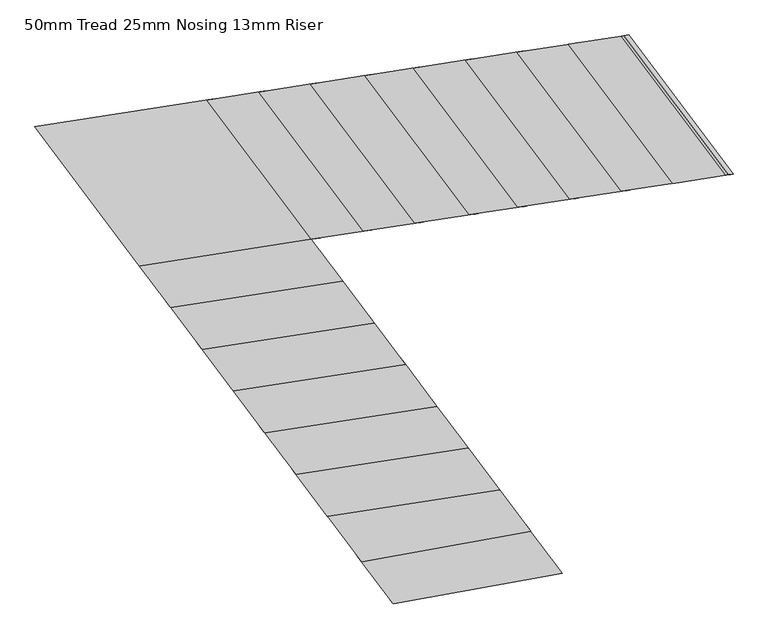
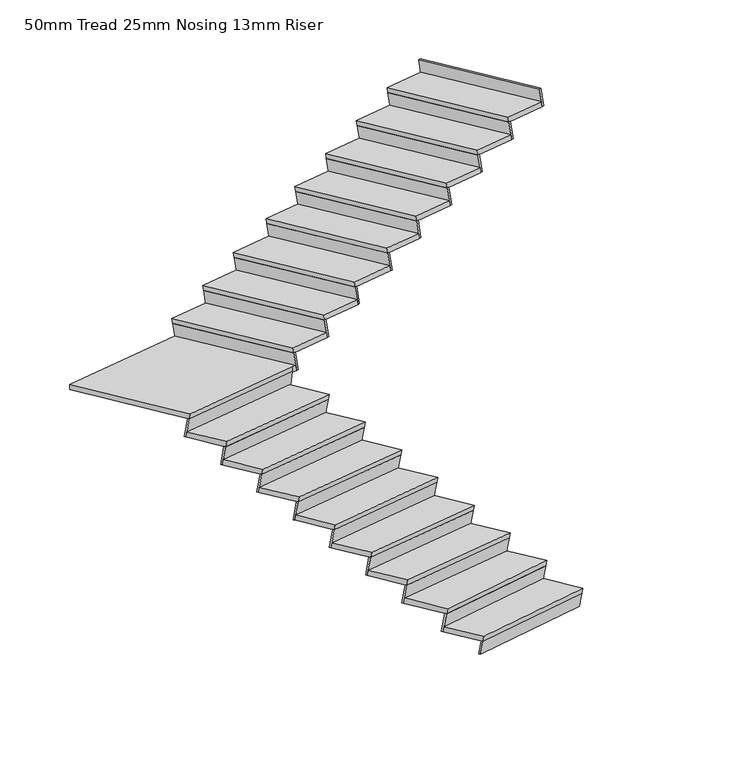
"""IFC4 building model written with IfcOpenShell, lengths in millimetres: stair flight geometry, 50mm Tread 25mm Nosing 13mm Riser."""

import ifcopenshell
import ifcopenshell.guid

model = None  # the IFC model being written
_history = None  # IfcOwnerHistory: only IFC2X3 demands one
_inside = {}  # id of a spatial element -> (the spatial element, [elements in it])
_under = {}  # id of a project, library or spatial element -> (it, [spatial elements below it])
_declared = {}  # id of a project -> (the project, [libraries it declares])
_typed = {}  # id of a type object -> (the type object, [elements of that type])
_made_of = {}  # id of a material, layer set ... -> (it, [elements and type objects made of it])


def new_model(schema):
    """Start an empty IFC model of exactly this schema.

    Asked for "IFC4X3", IfcOpenShell would pick the latest addendum, in which some entities
    have other attributes; the version numbers below select the first issue.
    IFC2X3 requires an IfcOwnerHistory on every rooted entity: one is made here for all.
    """
    global model, _history
    if schema == "IFC4X3":
        model = ifcopenshell.file(schema_version=(4, 3, 0, 0))
    else:
        model = ifcopenshell.file(schema=schema)
    _inside.clear()
    _under.clear()
    _declared.clear()
    _typed.clear()
    _made_of.clear()
    _history = None
    if model.schema == "IFC2X3":
        org = make("IfcOrganization", Name="unknown")
        user = make(
            "IfcPersonAndOrganization",
            ThePerson=make("IfcPerson", FamilyName="unknown"),
            TheOrganization=org,
        )
        app = make(
            "IfcApplication",
            ApplicationDeveloper=org,
            Version="unknown",
            ApplicationFullName="unknown",
            ApplicationIdentifier="unknown",
        )
        _history = make(
            "IfcOwnerHistory",
            OwningUser=user,
            OwningApplication=app,
            ChangeAction="ADDED",
            CreationDate=0,
        )
    return model


def make(cls, **values):
    """One entity of the class cls with the attributes given. An attribute that is None is left unset."""
    return model.create_entity(
        cls, **{name: value for name, value in values.items() if value is not None}
    )


def rooted(cls, **values):
    """An entity with a GlobalId (a new one), such as an element, a storey or a relation."""
    return make(cls, GlobalId=ifcopenshell.guid.new(), OwnerHistory=_history, **values)


def si_unit(unit_type, name, prefix=None):
    """IfcSIUnit, for example si_unit("LENGTHUNIT", "METRE", prefix="MILLI")."""
    return make("IfcSIUnit", UnitType=unit_type, Prefix=prefix, Name=name)


def assignment(units):
    """IfcUnitAssignment: the units of a project."""
    return None if units is None else make("IfcUnitAssignment", Units=units)


def point(xyz):
    """IfcCartesianPoint."""
    return None if xyz is None else make("IfcCartesianPoint", Coordinates=xyz)


def direction(xyz):
    """IfcDirection."""
    return None if xyz is None else make("IfcDirection", DirectionRatios=xyz)


def frame(location, z_axis=None, x_axis=None):
    """IfcAxis2Placement3D, a coordinate frame: its origin and axes. An axis left out is left unset."""
    return make(
        "IfcAxis2Placement3D",
        Location=point(location),
        Axis=direction(z_axis),
        RefDirection=direction(x_axis),
    )


def origin():
    """The frame at (0, 0, 0) with its axes left unset."""
    return frame((0.0, 0.0, 0.0))


def place(relative_to, where):
    """IfcLocalPlacement: puts the frame where relative to a parent placement (None: the world)."""
    return make(
        "IfcLocalPlacement", PlacementRelTo=relative_to, RelativePlacement=where
    )


def context(
    kind, dimensions, precision=None, world=None, true_north=None, identifier=None
):
    """IfcGeometricRepresentationContext, for example the 3D "Model" context."""
    return make(
        "IfcGeometricRepresentationContext",
        ContextIdentifier=identifier,
        ContextType=kind,
        CoordinateSpaceDimension=dimensions,
        Precision=precision,
        WorldCoordinateSystem=world,
        TrueNorth=true_north,
    )


def project(units=None, contexts=None):
    """IfcProject with its units and contexts."""
    return rooted(
        "IfcProject",
        Name="project",
        RepresentationContexts=contexts,
        UnitsInContext=assignment(units),
    )


def spatial(cls, under=None, at=None, **own):
    """A site, building, storey or space (cls), placed at a placement, below another one or the project."""
    s = rooted(cls, ObjectPlacement=at, **own)
    if under is not None:
        _under.setdefault(under.id(), (under, []))[1].append(s)
    return s


def faces_of(points, faces, orient=None, outer=None):
    """IfcFace entities. A face is a list of loops; a loop is a list of indices into points, from 0.

    orient and outer hold one flag for each loop. By default every Orientation is true, the
    first loop of a face is its IfcFaceOuterBound and the others are IfcFaceBound.
    """
    made = []
    for i, loops in enumerate(faces):
        bounds = []
        for j, loop in enumerate(loops):
            is_outer = j == 0 if outer is None else outer[i][j]
            bounds.append(
                make(
                    "IfcFaceOuterBound" if is_outer else "IfcFaceBound",
                    Bound=make("IfcPolyLoop", Polygon=[points[k] for k in loop]),
                    Orientation=True if orient is None else orient[i][j],
                )
            )
        made.append(make("IfcFace", Bounds=bounds))
    return made


def faceted_brep(points, faces, orient=None, outer=None, voids=None):
    """IfcFacetedBrep: a solid bounded by flat faces; with voids (closed shells), ...WithVoids."""
    shared = [point(p) for p in points]
    hull = make("IfcClosedShell", CfsFaces=faces_of(shared, faces, orient, outer))
    if voids is None:
        return make("IfcFacetedBrep", Outer=hull)
    return make(
        "IfcFacetedBrepWithVoids",
        Outer=hull,
        Voids=[
            make(cls, CfsFaces=faces_of(shared, fs, o, b)) for cls, fs, o, b in voids
        ],
    )


def shape(context_of_items, identifier, shape_type, items):
    """IfcShapeRepresentation: the items that make up one representation, for example the "Body"."""
    return make(
        "IfcShapeRepresentation",
        ContextOfItems=context_of_items,
        RepresentationIdentifier=identifier,
        RepresentationType=shape_type,
        Items=items,
    )


def source(mapping_origin, context_of_items, identifier, shape_type, items):
    """IfcRepresentationMap: a shape defined once, which mapped items show again and again."""
    return make(
        "IfcRepresentationMap",
        MappingOrigin=mapping_origin,
        MappedRepresentation=shape(context_of_items, identifier, shape_type, items),
    )


def transform(
    local_origin,
    x_axis=None,
    y_axis=None,
    z_axis=None,
    scale=None,
    scale2=None,
    scale3=None,
    uniform=True,
):
    """IfcCartesianTransformationOperator3D, or its non-uniform kind. x_axis, y_axis, z_axis: its Axis1, 2, 3."""
    if uniform:
        return make(
            "IfcCartesianTransformationOperator3D",
            Axis1=direction(x_axis),
            Axis2=direction(y_axis),
            LocalOrigin=point(local_origin),
            Scale=scale,
            Axis3=direction(z_axis),
        )
    return make(
        "IfcCartesianTransformationOperator3DnonUniform",
        Axis1=direction(x_axis),
        Axis2=direction(y_axis),
        LocalOrigin=point(local_origin),
        Scale=scale,
        Axis3=direction(z_axis),
        Scale2=scale2,
        Scale3=scale3,
    )


def mapped(mapping_source, mapping_target):
    """IfcMappedItem: shows the shape of a source again, moved by a transform."""
    return make(
        "IfcMappedItem", MappingSource=mapping_source, MappingTarget=mapping_target
    )


def made_of(thing, what):
    """Note that an element or type object is made of a material, layer set ...; save() writes the relation."""
    if what is not None:
        _made_of.setdefault(what.id(), (what, []))[1].append(thing)
    return thing


def element(
    cls,
    number,
    at=None,
    inside=None,
    cuts=None,
    type_object=None,
    material=None,
    context=None,
    identifier="Body",
    shape_type=None,
    held_by="IfcProductDefinitionShape",
    body=None,
    shapes=None,
    **own,
):
    """One element of the class cls, such as IfcWall. Its Tag is "e" and its number.

    at: its placement. inside: the storey or other place that contains it. cuts: it is an
    opening in that element (IfcRelVoidsElement). A single representation is given by context,
    identifier, shape_type and body (its items); several are given by shapes. held_by: the class
    of the entity that holds the representations. save() writes the other relations.
    """
    e = rooted(cls, Tag="e%d" % number, ObjectPlacement=at, **own)
    if body is not None:
        shapes = [shape(context, identifier, shape_type, body)]
    if shapes is not None:
        e.Representation = make(held_by, Representations=shapes)
    if inside is not None:
        _inside.setdefault(inside.id(), (inside, []))[1].append(e)
    if cuts is not None:
        rooted(
            "IfcRelVoidsElement", RelatingBuildingElement=cuts, RelatedOpeningElement=e
        )
    if type_object is not None:
        _typed.setdefault(type_object.id(), (type_object, []))[1].append(e)
    return made_of(e, material)


def aggregate(whole, parts):
    """IfcRelAggregates: a whole, such as a stair, and the parts it consists of."""
    return rooted("IfcRelAggregates", RelatingObject=whole, RelatedObjects=parts)


def save(model, path):
    """Write the relations noted so far, then the file.

    IfcRelAggregates (storeys below a building ...), IfcRelContainedInSpatialStructure (elements
    in a storey), IfcRelDefinesByType, IfcRelAssociatesMaterial and IfcRelDeclares: one each for
    every whole, place, type object, material and project.
    """
    for whole, parts in _under.values():
        aggregate(whole, parts)
    for where, things in _inside.values():
        rooted(
            "IfcRelContainedInSpatialStructure",
            RelatedElements=things,
            RelatingStructure=where,
        )
    for kind, things in _typed.values():
        rooted("IfcRelDefinesByType", RelatedObjects=things, RelatingType=kind)
    for what, things in _made_of.values():
        rooted("IfcRelAssociatesMaterial", RelatedObjects=things, RelatingMaterial=what)
    for by, libraries in _declared.values():
        rooted("IfcRelDeclares", RelatingContext=by, RelatedDefinitions=libraries)
    model.write(path)


def stair_flight_50mm_tread_25mm_nosing_13mm_riser_716ff132(model_context):
    return source(origin(), model_context, "Body", "Brep", [
        faceted_brep([(80293.6777293, 43226.6486407, 17175.0), (80288.8810609, 43233.0418362, 17125.0), (79317.3439262, 43057.8753097, 17125.0), (79322.1405946, 43051.4821142, 17175.0), (79518.9714946, 42789.1378561, 17175.0), (80490.5086293, 42964.3043826, 17175.0), (80485.7119608, 42970.6975781, 17125.0), (79514.1748261, 42795.5310516, 17125.0)], [[[0, 1, 2, 3]], [[3, 4, 5, 0]], [[2, 1, 6, 7]], [[4, 3, 2, 7]], [[0, 5, 6, 1]], [[5, 4, 7, 6]]]),
        faceted_brep([(80485.7119608, 42970.6975781, 17125.0), (80473.7202897, 42986.6805669, 17000.0), (80465.2408978, 42997.9822466, 17000.0), (80477.2325689, 42981.9992578, 17125.0), (79514.1748261, 42795.5310516, 17125.0), (79505.6954342, 42806.8327314, 17125.0), (79493.703763, 42822.8157201, 17000.0), (79502.183155, 42811.5140404, 17000.0)], [[[0, 1, 2, 3]], [[4, 5, 6, 7]], [[1, 0, 4, 7]], [[2, 1, 7, 6]], [[3, 2, 6, 5]], [[0, 3, 5, 4]]]),
        faceted_brep([(80305.6694004, 43210.6656519, 17300.0), (80288.8810609, 43233.0418362, 17125.0), (80280.4016689, 43244.3435159, 17125.0), (80297.1900085, 43221.9673316, 17300.0), (79334.1322657, 43035.4991254, 17300.0), (79325.6528738, 43046.8008052, 17300.0), (79308.8645342, 43069.1769895, 17125.0), (79317.3439262, 43057.8753097, 17125.0)], [[[0, 1, 2, 3]], [[4, 5, 6, 7]], [[1, 0, 4, 7]], [[2, 1, 7, 6]], [[3, 2, 6, 5]], [[0, 3, 5, 4]]]),
        faceted_brep([(79125.1762587, 43314.0042212, 17350.0), (79338.9289342, 43029.1059299, 17350.0), (80310.4660689, 43204.2724564, 17350.0), (80113.4175257, 43466.9067982, 17350.0), (79120.3174064, 43320.4802978, 17300.0), (80108.5586735, 43473.3828748, 17300.0), (80305.6694004, 43210.6656519, 17300.0), (79334.1322657, 43035.4991254, 17300.0)], [[[0, 1, 2, 3]], [[4, 5, 6, 7]], [[1, 0, 4, 7]], [[3, 2, 6, 5]], [[3, 5, 4, 0]], [[2, 1, 7, 6]]]),
        faceted_brep([(80125.5646563, 43450.7166068, 17475.0), (80108.5586735, 43473.3828748, 17300.0), (80099.9693551, 43484.8310689, 17300.0), (80116.9753379, 43462.1648009, 17475.0), (79137.3233892, 43297.8140298, 17475.0), (79128.7340708, 43309.2622239, 17475.0), (79111.7280881, 43331.9284919, 17300.0), (79120.3174064, 43320.4802978, 17300.0)], [[[0, 1, 2, 3]], [[4, 5, 6, 7]], [[1, 0, 4, 7]], [[2, 1, 7, 6]], [[3, 2, 6, 5]], [[0, 3, 5, 4]]]),
        faceted_brep([(78945.1336983, 43553.972295, 17525.0), (79142.1822414, 43291.3379532, 17525.0), (80130.4235085, 43444.2405302, 17525.0), (79933.3749653, 43706.874872, 17525.0), (78940.274846, 43560.4483716, 17475.0), (79928.5161131, 43713.3509486, 17475.0), (80125.5646563, 43450.7166068, 17475.0), (79137.3233892, 43297.8140298, 17475.0)], [[[0, 1, 2, 3]], [[4, 5, 6, 7]], [[1, 0, 4, 7]], [[3, 2, 6, 5]], [[3, 5, 4, 0]], [[2, 1, 7, 6]]]),
        faceted_brep([(79945.5220959, 43690.6846806, 17650.0), (79928.5161131, 43713.3509486, 17475.0), (79919.9267947, 43724.7991427, 17475.0), (79936.9327775, 43702.1328747, 17650.0), (78957.2808288, 43537.7821036, 17650.0), (78948.6915104, 43549.2302977, 17650.0), (78931.6855277, 43571.8965657, 17475.0), (78940.274846, 43560.4483716, 17475.0)], [[[0, 1, 2, 3]], [[4, 5, 6, 7]], [[1, 0, 4, 7]], [[2, 1, 7, 6]], [[3, 2, 6, 5]], [[0, 3, 5, 4]]]),
        faceted_brep([(78765.0911379, 43793.9403688, 17700.0), (78962.139681, 43531.306027, 17700.0), (79950.3809481, 43684.208604, 17700.0), (79753.3324049, 43946.8429458, 17700.0), (78760.2322857, 43800.4164454, 17650.0), (79748.4735527, 43953.3190224, 17650.0), (79945.5220959, 43690.6846806, 17650.0), (78957.2808288, 43537.7821036, 17650.0)], [[[0, 1, 2, 3]], [[4, 5, 6, 7]], [[1, 0, 4, 7]], [[3, 2, 6, 5]], [[3, 5, 4, 0]], [[2, 1, 7, 6]]]),
        faceted_brep([(79765.4795355, 43930.6527544, 17825.0), (79748.4735527, 43953.3190224, 17650.0), (79739.8842343, 43964.7672165, 17650.0), (79756.8902171, 43942.1009485, 17825.0), (78777.2382684, 43777.7501774, 17825.0), (78768.64895, 43789.1983715, 17825.0), (78751.6429673, 43811.8646395, 17650.0), (78760.2322857, 43800.4164454, 17650.0)], [[[0, 1, 2, 3]], [[4, 5, 6, 7]], [[1, 0, 4, 7]], [[2, 1, 7, 6]], [[3, 2, 6, 5]], [[0, 3, 5, 4]]]),
        faceted_brep([(78585.0485775, 44033.9084426, 17875.0), (78782.0971206, 43771.2741008, 17875.0), (79770.3383877, 43924.1766778, 17875.0), (79573.2898445, 44186.8110196, 17875.0), (78580.1897253, 44040.3845192, 17825.0), (79568.4309923, 44193.2870962, 17825.0), (79765.4795355, 43930.6527544, 17825.0), (78777.2382684, 43777.7501774, 17825.0)], [[[0, 1, 2, 3]], [[4, 5, 6, 7]], [[1, 0, 4, 7]], [[3, 2, 6, 5]], [[3, 5, 4, 0]], [[2, 1, 7, 6]]]),
        faceted_brep([(79585.4369751, 44170.6208282, 18000.0), (79568.4309923, 44193.2870962, 17825.0), (79559.841674, 44204.7352904, 17825.0), (79576.8476567, 44182.0690223, 18000.0), (78597.195708, 44017.7182512, 18000.0), (78588.6063896, 44029.1664453, 18000.0), (78571.6004069, 44051.8327134, 17825.0), (78580.1897253, 44040.3845192, 17825.0)], [[[0, 1, 2, 3]], [[4, 5, 6, 7]], [[1, 0, 4, 7]], [[2, 1, 7, 6]], [[3, 2, 6, 5]], [[0, 3, 5, 4]]]),
        faceted_brep([(78405.0060171, 44273.8765164, 18050.0), (78602.0545602, 44011.2421746, 18050.0), (79590.2958273, 44164.1447516, 18050.0), (79393.2472842, 44426.7790934, 18050.0), (78400.1471649, 44280.352593, 18000.0), (79388.3884319, 44433.25517, 18000.0), (79585.4369751, 44170.6208282, 18000.0), (78597.195708, 44017.7182512, 18000.0)], [[[0, 1, 2, 3]], [[4, 5, 6, 7]], [[1, 0, 4, 7]], [[3, 2, 6, 5]], [[3, 5, 4, 0]], [[2, 1, 7, 6]]]),
        faceted_brep([(79405.3944147, 44410.588902, 18175.0), (79388.3884319, 44433.25517, 18000.0), (79379.7991136, 44444.7033642, 18000.0), (79396.8050963, 44422.0370962, 18175.0), (78417.1531476, 44257.686325, 18175.0), (78408.5638292, 44269.1345192, 18175.0), (78391.5578465, 44291.8007872, 18000.0), (78400.1471649, 44280.352593, 18000.0)], [[[0, 1, 2, 3]], [[4, 5, 6, 7]], [[1, 0, 4, 7]], [[2, 1, 7, 6]], [[3, 2, 6, 5]], [[0, 3, 5, 4]]]),
        faceted_brep([(78224.9634567, 44513.8445902, 18225.0), (78422.0119998, 44251.2102484, 18225.0), (79410.2532669, 44404.1128254, 18225.0), (79213.2047238, 44666.7471672, 18225.0), (78220.1046045, 44520.3206668, 18175.0), (79208.3458715, 44673.2232438, 18175.0), (79405.3944147, 44410.588902, 18175.0), (78417.1531476, 44257.686325, 18175.0)], [[[0, 1, 2, 3]], [[4, 5, 6, 7]], [[1, 0, 4, 7]], [[3, 2, 6, 5]], [[3, 5, 4, 0]], [[2, 1, 7, 6]]]),
        faceted_brep([(79225.3518543, 44650.5569758, 18350.0), (79208.3458715, 44673.2232438, 18175.0), (79199.7565532, 44684.671438, 18175.0), (79216.7625359, 44662.00517, 18350.0), (78237.1105872, 44497.6543988, 18350.0), (78228.5212688, 44509.102593, 18350.0), (78211.5152861, 44531.768861, 18175.0), (78220.1046045, 44520.3206668, 18175.0)], [[[0, 1, 2, 3]], [[4, 5, 6, 7]], [[1, 0, 4, 7]], [[2, 1, 7, 6]], [[3, 2, 6, 5]], [[0, 3, 5, 4]]]),
        faceted_brep([(78044.9208963, 44753.812664, 18400.0), (78241.9694394, 44491.1783222, 18400.0), (79230.2107065, 44644.0808992, 18400.0), (79033.1621634, 44906.715241, 18400.0), (78040.0620441, 44760.2887406, 18350.0), (79028.3033111, 44913.1913176, 18350.0), (79225.3518543, 44650.5569758, 18350.0), (78237.1105872, 44497.6543988, 18350.0)], [[[0, 1, 2, 3]], [[4, 5, 6, 7]], [[1, 0, 4, 7]], [[3, 2, 6, 5]], [[3, 5, 4, 0]], [[2, 1, 7, 6]]]),
        faceted_brep([(79049.0759849, 44891.1078392, 18525.0), (79045.2534204, 44915.8138709, 18350.0), (79043.3227338, 44928.2923013, 18350.0), (79047.1452983, 44903.5862696, 18525.0), (78057.0680268, 44737.6224726, 18525.0), (78048.4787085, 44749.0706668, 18525.0), (78031.4727257, 44771.7369348, 18350.0), (78040.0620441, 44760.2887406, 18350.0)], [[[0, 1, 2, 3]], [[4, 5, 6, 7]], [[1, 0, 4, 7]], [[2, 1, 7, 6]], [[3, 2, 6, 5]], [[0, 3, 5, 4]]]),
        faceted_brep([(78478.0296801, 45688.2752923, 18575.0), (77461.7850111, 45531.0399754, 18575.0), (78061.926879, 44731.146396, 18575.0), (79050.1681461, 44884.048973, 18575.0), (79078.1715481, 44888.3817129, 18575.0), (78486.0306521, 45689.5132179, 18525.0), (79086.17252, 44889.6196386, 18525.0), (79050.1681461, 44884.048973, 18525.0), (79049.0759849, 44891.1078392, 18525.0), (78057.0680268, 44737.6224726, 18525.0), (77461.7850111, 45531.0399754, 18525.0)], [[[0, 1, 2, 3, 4]], [[5, 6, 7, 8, 9, 10]], [[1, 0, 5, 10]], [[2, 1, 10, 9]], [[4, 3, 7, 6]], [[4, 6, 5, 0]], [[3, 8, 7]], [[8, 3, 2, 9]]]),
        faceted_brep([(79058.1691181, 44885.2868987, 18700.0), (79086.17252, 44889.6196386, 18525.0), (79100.3163739, 44891.8080027, 18525.0), (79072.312972, 44887.4752628, 18700.0), (78458.0272501, 45685.1804781, 18700.0), (78472.171104, 45687.3688422, 18700.0), (78500.1745059, 45691.701582, 18525.0), (78486.0306521, 45689.5132179, 18525.0)], [[[0, 1, 2, 3]], [[4, 5, 6, 7]], [[1, 0, 4, 7]], [[2, 1, 7, 6]], [[3, 2, 6, 5]], [[0, 3, 5, 4]]]),
        faceted_brep([(78774.5020602, 45734.1460654, 18750.0), (78450.0262781, 45683.9425524, 18750.0), (79050.1681461, 44884.048973, 18750.0), (79374.6439282, 44934.252486, 18750.0), (78782.5030322, 45735.383991, 18700.0), (79382.6449002, 44935.4904117, 18700.0), (79058.1691181, 44885.2868987, 18700.0), (78458.0272501, 45685.1804781, 18700.0)], [[[0, 1, 2, 3]], [[4, 5, 6, 7]], [[1, 0, 4, 7]], [[3, 2, 6, 5]], [[3, 5, 4, 0]], [[2, 1, 7, 6]]]),
        faceted_brep([(79354.6414982, 44931.1576718, 18875.0), (79382.6449002, 44935.4904117, 18700.0), (79396.788754, 44937.6787758, 18700.0), (79368.7853521, 44933.3460359, 18875.0), (78754.4996302, 45731.0512512, 18875.0), (78768.6434841, 45733.2396153, 18875.0), (78796.646886, 45737.5723551, 18700.0), (78782.5030322, 45735.383991, 18700.0)], [[[0, 1, 2, 3]], [[4, 5, 6, 7]], [[1, 0, 4, 7]], [[2, 1, 7, 6]], [[3, 2, 6, 5]], [[0, 3, 5, 4]]]),
        faceted_brep([(79070.9744403, 45780.0168385, 18925.0), (78746.4986583, 45729.8133255, 18925.0), (79346.6405262, 44929.9197461, 18925.0), (79671.1163083, 44980.1232591, 18925.0), (79078.9754123, 45781.2547641, 18875.0), (79679.1172803, 44981.3611848, 18875.0), (79354.6414982, 44931.1576718, 18875.0), (78754.4996302, 45731.0512512, 18875.0)], [[[0, 1, 2, 3]], [[4, 5, 6, 7]], [[1, 0, 4, 7]], [[3, 2, 6, 5]], [[3, 5, 4, 0]], [[2, 1, 7, 6]]]),
        faceted_brep([(79651.1138783, 44977.0284449, 19050.0), (79679.1172803, 44981.3611848, 18875.0), (79693.2611341, 44983.5495489, 18875.0), (79665.2577322, 44979.216809, 19050.0), (79050.9720104, 45776.9220243, 19050.0), (79065.1158642, 45779.1103884, 19050.0), (79093.1192662, 45783.4431282, 18875.0), (79078.9754123, 45781.2547641, 18875.0)], [[[0, 1, 2, 3]], [[4, 5, 6, 7]], [[1, 0, 4, 7]], [[2, 1, 7, 6]], [[3, 2, 6, 5]], [[0, 3, 5, 4]]]),
        faceted_brep([(79385.5810477, 45828.6933738, 19100.0), (79042.9710384, 45775.6840986, 19100.0), (79643.1129064, 44975.7905192, 19100.0), (79985.7229157, 45028.7997945, 19100.0), (79393.5820197, 45829.9312995, 19050.0), (79993.7238877, 45030.0377202, 19050.0), (79651.1138783, 44977.0284449, 19050.0), (79050.9720104, 45776.9220243, 19050.0)], [[[0, 1, 2, 3]], [[4, 5, 6, 7]], [[1, 0, 4, 7]], [[3, 2, 6, 5]], [[3, 5, 4, 0]], [[2, 1, 7, 6]]]),
        faceted_brep([(79965.7204857, 45025.7049803, 19225.0), (79993.7238877, 45030.0377202, 19050.0), (80007.8677415, 45032.2260843, 19050.0), (79979.8643396, 45027.8933444, 19225.0), (79365.5786177, 45825.5985597, 19225.0), (79379.7224716, 45827.7869238, 19225.0), (79407.7258735, 45832.1196636, 19050.0), (79393.5820197, 45829.9312995, 19050.0)], [[[0, 1, 2, 3]], [[4, 5, 6, 7]], [[1, 0, 4, 7]], [[2, 1, 7, 6]], [[3, 2, 6, 5]], [[0, 3, 5, 4]]]),
        faceted_brep([(79663.9192006, 45871.7583847, 19275.0), (79357.5776457, 45824.360634, 19275.0), (79957.7195137, 45024.4670546, 19275.0), (80264.0610685, 45071.8648053, 19275.0), (79671.9201725, 45872.9963103, 19225.0), (80272.0620405, 45073.102731, 19225.0), (79965.7204857, 45025.7049803, 19225.0), (79365.5786177, 45825.5985597, 19225.0)], [[[0, 1, 2, 3]], [[4, 5, 6, 7]], [[1, 0, 4, 7]], [[3, 2, 6, 5]], [[3, 5, 4, 0]], [[2, 1, 7, 6]]]),
        faceted_brep([(80244.0586386, 45068.7699911, 19400.0), (80272.0620405, 45073.102731, 19225.0), (80286.2058944, 45075.2910951, 19225.0), (80258.2024925, 45070.9583552, 19400.0), (79643.9167706, 45868.6635705, 19400.0), (79658.0606245, 45870.8519346, 19400.0), (79686.0640264, 45875.1846744, 19225.0), (79671.9201725, 45872.9963103, 19225.0)], [[[0, 1, 2, 3]], [[4, 5, 6, 7]], [[1, 0, 4, 7]], [[2, 1, 7, 6]], [[3, 2, 6, 5]], [[0, 3, 5, 4]]]),
        faceted_brep([(79960.3915807, 45917.6291578, 19450.0), (79635.9157986, 45867.4256448, 19450.0), (80236.0576666, 45067.5320654, 19450.0), (80560.5334487, 45117.7355784, 19450.0), (79968.3925527, 45918.8670834, 19400.0), (80568.5344207, 45118.9735041, 19400.0), (80244.0586386, 45068.7699911, 19400.0), (79643.9167706, 45868.6635705, 19400.0)], [[[0, 1, 2, 3]], [[4, 5, 6, 7]], [[1, 0, 4, 7]], [[3, 2, 6, 5]], [[3, 5, 4, 0]], [[2, 1, 7, 6]]]),
        faceted_brep([(80540.5310187, 45114.6407642, 19575.0), (80568.5344207, 45118.9735041, 19400.0), (80582.6782745, 45121.1618682, 19400.0), (80554.6748726, 45116.8291283, 19575.0), (79940.3891507, 45914.5343436, 19575.0), (79954.5330046, 45916.7227077, 19575.0), (79982.5364065, 45921.0554475, 19400.0), (79968.3925527, 45918.8670834, 19400.0)], [[[0, 1, 2, 3]], [[4, 5, 6, 7]], [[1, 0, 4, 7]], [[2, 1, 7, 6]], [[3, 2, 6, 5]], [[0, 3, 5, 4]]]),
        faceted_brep([(80256.8639608, 45963.4999309, 19625.0), (79932.3881787, 45913.2964179, 19625.0), (80532.5300467, 45113.4028386, 19625.0), (80857.0058288, 45163.6063515, 19625.0), (80264.8649328, 45964.7378565, 19575.0), (80865.0068008, 45164.8442772, 19575.0), (80540.5310187, 45114.6407642, 19575.0), (79940.3891507, 45914.5343436, 19575.0)], [[[0, 1, 2, 3]], [[4, 5, 6, 7]], [[1, 0, 4, 7]], [[3, 2, 6, 5]], [[3, 5, 4, 0]], [[2, 1, 7, 6]]]),
        faceted_brep([(80837.0033988, 45160.5115373, 19750.0), (80865.0068008, 45164.8442772, 19575.0), (80879.1506546, 45167.0326413, 19575.0), (80851.1472527, 45162.6999014, 19750.0), (80236.8615308, 45960.4051167, 19750.0), (80251.0053847, 45962.5934808, 19750.0), (80279.0087866, 45966.9262206, 19575.0), (80264.8649328, 45964.7378565, 19575.0)], [[[0, 1, 2, 3]], [[4, 5, 6, 7]], [[1, 0, 4, 7]], [[2, 1, 7, 6]], [[3, 2, 6, 5]], [[0, 3, 5, 4]]]),
        faceted_brep([(80553.3363409, 46009.370704, 19800.0), (80228.8605589, 45959.167191, 19800.0), (80829.0024268, 45159.2736117, 19800.0), (81153.4782089, 45209.4771246, 19800.0), (80561.3373129, 46010.6086296, 19750.0), (81161.4791809, 45210.7150503, 19750.0), (80837.0033988, 45160.5115373, 19750.0), (80236.8615308, 45960.4051167, 19750.0)], [[[0, 1, 2, 3]], [[4, 5, 6, 7]], [[1, 0, 4, 7]], [[3, 2, 6, 5]], [[3, 5, 4, 0]], [[2, 1, 7, 6]]]),
        faceted_brep([(81133.475779, 45206.3823104, 19925.0), (81161.4791809, 45210.7150503, 19750.0), (81175.6230348, 45212.9034144, 19750.0), (81147.6196328, 45208.5706745, 19925.0), (80533.333911, 46006.2758898, 19925.0), (80547.4777648, 46008.4642539, 19925.0), (80575.4811668, 46012.7969937, 19750.0), (80561.3373129, 46010.6086296, 19750.0)], [[[0, 1, 2, 3]], [[4, 5, 6, 7]], [[1, 0, 4, 7]], [[2, 1, 7, 6]], [[3, 2, 6, 5]], [[0, 3, 5, 4]]]),
        faceted_brep([(81429.9481591, 45252.2530835, 20100.0), (81457.951561, 45256.5858234, 19925.0), (81472.0954149, 45258.7741875, 19925.0), (81444.0920129, 45254.4414476, 20100.0), (80829.8062911, 46052.1466629, 20100.0), (80843.950145, 46054.335027, 20100.0), (80871.9535469, 46058.6677668, 19925.0), (80857.809693, 46056.4794027, 19925.0)], [[[0, 1, 2, 3]], [[4, 5, 6, 7]], [[1, 0, 4, 7]], [[2, 1, 7, 6]], [[3, 2, 6, 5]], [[0, 3, 5, 4]]]),
        faceted_brep([(80849.808721, 46055.2414771, 19975.0), (80525.332939, 46005.0379641, 19975.0), (81125.474807, 45205.1443848, 19975.0), (81449.950589, 45255.3478977, 19975.0), (80857.809693, 46056.4794027, 19925.0), (81457.951561, 45256.5858234, 19925.0), (81133.475779, 45206.3823104, 19925.0), (80533.333911, 46006.2758898, 19925.0)], [[[0, 1, 2, 3]], [[4, 5, 6, 7]], [[1, 0, 4, 7]], [[3, 2, 6, 5]], [[3, 5, 4, 0]], [[2, 1, 7, 6]]]),
    ])


if __name__ == "__main__":
    model = new_model("IFC4")
    model_context = context("Model", 3, world=origin())
    ifc_project = project(units=[si_unit("LENGTHUNIT", "METRE", prefix="MILLI")], contexts=[model_context])
    site = spatial("IfcSite", under=ifc_project)
    building = spatial("IfcBuilding", under=site)
    placement = place(None, origin())
    stair_flight_50mm_tread_25mm_nosing_13mm_riser_shape = stair_flight_50mm_tread_25mm_nosing_13mm_riser_716ff132(model_context)
    element("IfcStairFlight", 1, ObjectType="50mm Tread 25mm Nosing 13mm Riser", at=placement, inside=building, context=model_context, shape_type="MappedRepresentation", body=[
        mapped(stair_flight_50mm_tread_25mm_nosing_13mm_riser_shape, transform((0.0, 0.0, 0.0), x_axis=(1.0, 0.0, 0.0), y_axis=(0.0, 1.0, 0.0), z_axis=(0.0, 0.0, 1.0))),
    ])
    save(model, "model.ifc")
